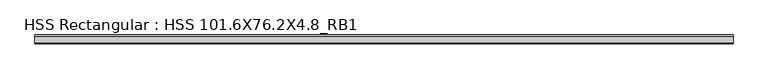
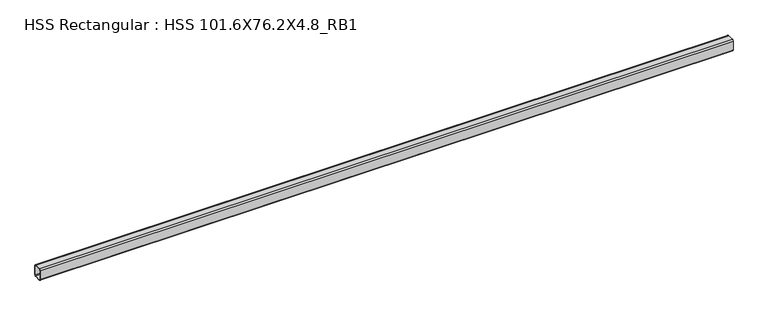
"""IFC4 building model written with IfcOpenShell, lengths in millimetres: beam geometry, HSS Rectangular : HSS 101.6X76.2X4.8_RB1."""

from ifc_helpers import new_model, si_unit, point, frame, frame_2d, origin, place, context, project, spatial, polyline, circle_curve, trimmed, segment, composite_curve, outline, extrude, source, transform, mapped, element, save


def hss_rectangular_hss_101_6x76_2x4_8_rb1_2247a570(model_context):
    return source(origin(), model_context, "Body", "SweptSolid", [
        extrude(outline(composite_curve([segment(polyline([(38.1, 41.275), (38.1, -41.275)]), True, "CONTINUOUS"), segment(trimmed(circle_curve(frame_2d((28.575, -41.275)), 9.525), [point((38.1, -41.275))], [point((28.575, -50.8))], False, "CARTESIAN"), True, "CONTINUOUS"), segment(polyline([(28.575, -50.8), (-28.575, -50.8)]), True, "CONTINUOUS"), segment(trimmed(circle_curve(frame_2d((-28.575, -41.275)), 9.525), [point((-28.575, -50.8))], [point((-38.1, -41.275))], False, "CARTESIAN"), True, "CONTINUOUS"), segment(polyline([(-38.1, -41.275), (-38.1, 41.275)]), True, "CONTINUOUS"), segment(trimmed(circle_curve(frame_2d((-28.575, 41.275)), 9.525), [point((-38.1, 41.275))], [point((-28.575, 50.8))], False, "CARTESIAN"), True, "CONTINUOUS"), segment(polyline([(-28.575, 50.8), (28.575, 50.8)]), True, "CONTINUOUS"), segment(trimmed(circle_curve(frame_2d((28.575, 41.275)), 9.525), [point((28.575, 50.8))], [point((38.1, 41.275))], False, "CARTESIAN"), True, "CONTINUOUS")], self_intersect=False), holes=[composite_curve([segment(trimmed(circle_curve(frame_2d((-28.575, 41.275)), 4.7625), [point((-28.575, 46.0375))], [point((-33.3375, 41.275))], True, "CARTESIAN"), True, "CONTINUOUS"), segment(polyline([(-33.3375, 41.275), (-33.3375, -41.275)]), True, "CONTINUOUS"), segment(trimmed(circle_curve(frame_2d((-28.575, -41.275)), 4.7625), [point((-33.3375, -41.275))], [point((-28.575, -46.0375))], True, "CARTESIAN"), True, "CONTINUOUS"), segment(polyline([(-28.575, -46.0375), (28.575, -46.0375)]), True, "CONTINUOUS"), segment(trimmed(circle_curve(frame_2d((28.575, -41.275)), 4.7625), [point((28.575, -46.0375))], [point((33.3375, -41.275))], True, "CARTESIAN"), True, "CONTINUOUS"), segment(polyline([(33.3375, -41.275), (33.3375, 41.275)]), True, "CONTINUOUS"), segment(trimmed(circle_curve(frame_2d((28.575, 41.275)), 4.7625), [point((33.3375, 41.275))], [point((28.575, 46.0375))], True, "CARTESIAN"), True, "CONTINUOUS"), segment(polyline([(28.575, 46.0375), (-28.575, 46.0375)]), True, "CONTINUOUS")], self_intersect=False)]), frame((-7500.0, 0.0, 0.0), z_axis=(1.0, 0.0, 0.0), x_axis=(0.0, 1.0, 0.0)), (0.0, 0.0, 1.0), 5961.054677),
    ])


if __name__ == "__main__":
    model = new_model("IFC4")
    model_context = context("Model", 3, world=origin())
    ifc_project = project(units=[si_unit("LENGTHUNIT", "METRE", prefix="MILLI")], contexts=[model_context])
    site = spatial("IfcSite", under=ifc_project)
    building = spatial("IfcBuilding", under=site)
    placement = place(None, origin())
    hss_rectangular_hss_101_6x76_2x4_8_rb1_shape = hss_rectangular_hss_101_6x76_2x4_8_rb1_2247a570(model_context)
    element("IfcBeam", 1, ObjectType="HSS Rectangular : HSS 101.6X76.2X4.8_RB1", at=placement, inside=building, context=model_context, shape_type="MappedRepresentation", body=[
        mapped(hss_rectangular_hss_101_6x76_2x4_8_rb1_shape, transform((0.0, 0.0, 0.0), x_axis=(1.0, 0.0, 0.0), y_axis=(0.0, 1.0, 0.0), z_axis=(0.0, 0.0, 1.0))),
    ])
    save(model, "model.ifc")

# Revit data of these elements
# Type "HSS Rectangular : HSS 101.6X76.2X4.8_RB1"
#   Section Name Key = "HSS 4X3X3/16"
#   Assembly Code = "B10"
#   Width = 7.62 cm
#   Wall Nominal Thickness = 0.4763 cm
#   Wall Design Thickness = 0.442 cm
#   Torsional Moment of Inertia = 260.561 cm⁴
#   Torsional Modulus = 61.2876 cm³
#   Section Area = 14.4516 cm²
#   Plastic Modulus weak axis = 40.3122 cm³
#   Plastic Modulus strong axis = 49.1612 cm³
#   Perimeter = 0.881482 m²/m
#   Outer Fillet = 0.9525 cm
#   Nominal Weight = 12.1285 kgf/m
#   Moment of Inertia weak axis = 131.529 cm⁴
#   Moment of Inertia strong axis = 205.202 cm⁴
#   Inner Fillet = 0.4763 cm
#   Height = 10.16 cm
#   Elastic Modulus weak axis = 34.4128 cm³
#   Elastic Modulus strong axis = 40.476 cm³
#   Centroid Vertical = 5.08 cm
#   Centroid Horizontal = 3.81 cm
#   Length [instance default] = 1524 mm
#   Structural Material [instance default] = Steel ASTM A500, Grade B, Rectangular and Square
#   Principal Axes Angle = 0
# Element 1 (IfcBeam, "HSS Rectangular : HSS 101.6X76.2X4.8_RB1")
#   Structural Material = Steel ASTM A992
#   Materials on its faces: "Steel ASTM A992"
# Materials
#   "Steel ASTM A500, Grade B, Rectangular and Square": class "Metal", colour RGB 199 199 199, transparency 0, Description = "Carbon steel", Cost = 0
#   "Steel ASTM A992": class "Metal", colour RGB 199 199 199, transparency 0, Description = "Structural steel 50ksi", Cost = 0
